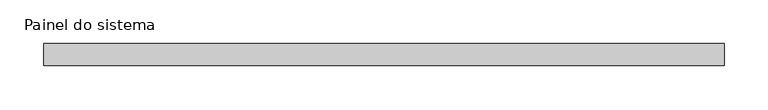
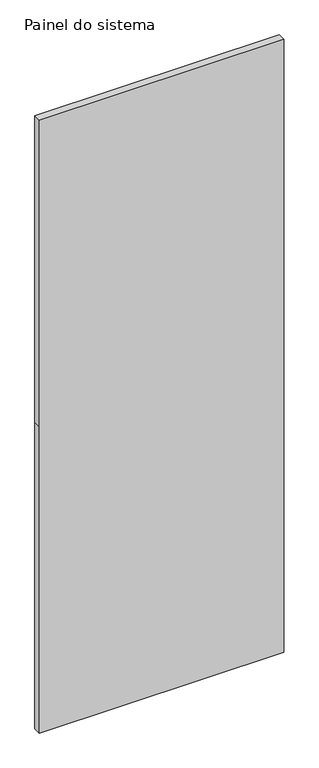
"""IFC4 building model written with IfcOpenShell, lengths in millimetres: plate geometry, Painel do sistema : Envidraçado."""

from ifc_helpers import new_model, si_unit, frame, origin, place, context, project, spatial, polyline, outline, extrude, source, transform, mapped, element, save


def painel_do_sistema_ee460c7a(model_context):
    return source(origin(), model_context, "Body", "SweptSolid", [
        extrude(outline(polyline([(0.0, -386.4083333), (0.0, 386.4083333), (1025.0, 386.4083333), (2050.0, 386.4083333), (2050.0, -386.4083333), (1025.0, -386.4083333), (0.0, -386.4083333)])), frame((0.0, -49.5, 0.0), z_axis=(0.0, 1.0, 0.0), x_axis=(0.0, 0.0, 1.0)), (0.0, 0.0, 1.0), 25.0),
    ])


if __name__ == "__main__":
    model = new_model("IFC4")
    model_context = context("Model", 3, world=origin())
    ifc_project = project(units=[si_unit("LENGTHUNIT", "METRE", prefix="MILLI")], contexts=[model_context])
    site = spatial("IfcSite", under=ifc_project)
    building = spatial("IfcBuilding", under=site)
    placement = place(None, origin())
    painel_do_sistema_shape = painel_do_sistema_ee460c7a(model_context)
    element("IfcPlate", 1, ObjectType="Painel do sistema : Envidraçado", at=placement, inside=building, context=model_context, shape_type="MappedRepresentation", body=[
        mapped(painel_do_sistema_shape, transform((0.0, 0.0, 0.0), x_axis=(1.0, 0.0, 0.0), y_axis=(0.0, 1.0, 0.0), z_axis=(0.0, 0.0, 1.0))),
    ])
    save(model, "model.ifc")

# Revit data of these elements
# Type "Painel do sistema : Envidraçado"
#   Construction Type Id = "GSP4R"
#   Analytic Construction = "Vidraça única Pilkington 1/8 pol"
#   Visual Light Transmittance = 0.9
#   Solar Heat Gain Coefficient = 0.86
#   Heat Transfer Coefficient (U) = 6.7069 W/(m²·K)
# Element 1 (IfcPlate, "Painel do sistema : Envidraçado")
#   Materials on its faces: ".VIDRO GENÉRICO"
# Materials
#   ".VIDRO GENÉRICO": class ".CC_VIDRO", colour RGB 0 128 192, transparency 0.9, Description = "Vidro comum", Cost = 0
